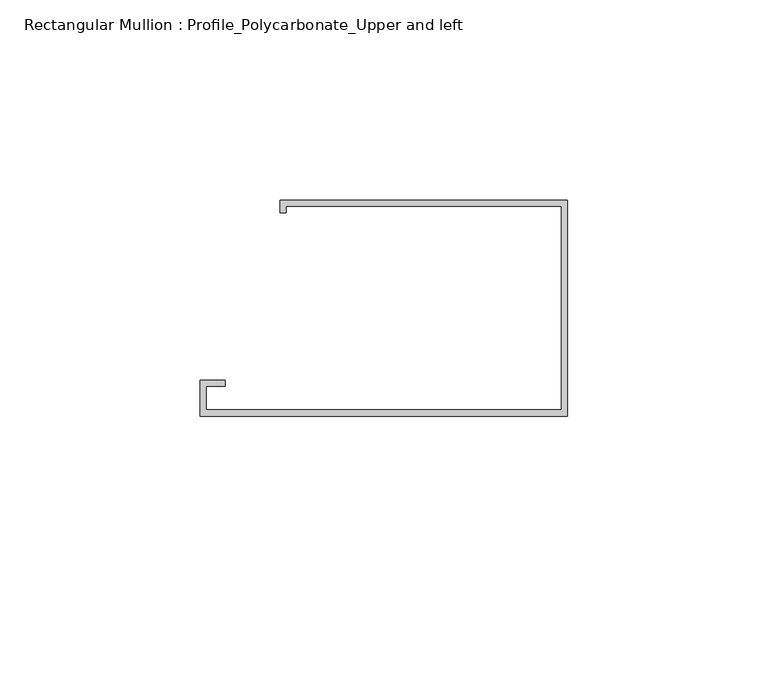
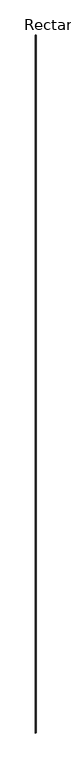
"""IFC4 building model written with IfcOpenShell, lengths in millimetres: member geometry, Rectangular Mullion : Profile_Polycarbonate_Upper and left."""

from ifc_helpers import new_model, si_unit, frame, origin, place, context, project, spatial, polyline, outline, extrude, source, transform, mapped, element, save


def rectangular_mullion_profile_polycarbonate_upper_and_left_29eb8ea6(model_context):
    return source(origin(), model_context, "Body", "SweptSolid", [
        extrude(outline(polyline([(0.0, -28.984575), (-91.9988, -28.984575), (-91.9988, -19.992975), (-85.6488, -19.992975), (-85.6488, -21.580475), (-90.4113, -21.580475), (-90.4113, -27.397075), (-1.5875, -27.397075), (-1.5875, 23.428325), (-70.3961, 23.428325), (-70.3961, 21.840825), (-71.9836, 21.840825), (-71.9836, 25.015825), (0.0, 25.015825), (0.0, -28.984575)])), frame((0.0, 0.0, -81480.3315463), z_axis=(0.0, 0.0, 1.0), x_axis=(1.0, 0.0, 0.0)), (0.0, 0.0, 1.0), 81480.3315463),
    ])


if __name__ == "__main__":
    model = new_model("IFC4")
    model_context = context("Model", 3, world=origin())
    ifc_project = project(units=[si_unit("LENGTHUNIT", "METRE", prefix="MILLI")], contexts=[model_context])
    site = spatial("IfcSite", under=ifc_project)
    building = spatial("IfcBuilding", under=site)
    placement = place(None, origin())
    rectangular_mullion_profile_polycarbonate_upper_and_left_shape = rectangular_mullion_profile_polycarbonate_upper_and_left_29eb8ea6(model_context)
    element("IfcMember", 1, ObjectType="Rectangular Mullion : Profile_Polycarbonate_Upper and left", at=placement, inside=building, context=model_context, shape_type="MappedRepresentation", body=[
        mapped(rectangular_mullion_profile_polycarbonate_upper_and_left_shape, transform((0.0, 0.0, 0.0), x_axis=(1.0, 0.0, 0.0), y_axis=(0.0, 1.0, 0.0), z_axis=(0.0, 0.0, 1.0))),
    ])
    save(model, "model.ifc")

# Revit data of these elements
# Type "Rectangular Mullion : Profile_Polycarbonate_Upper and left"
#   built-in parameter 1007322 = 0.177167 (stored number, unit not read)
#   built-in parameter 1007321 = 0.00520833 (stored number, unit not read)
#   built-in parameter 1007320 = 0 (stored number, unit not read)
